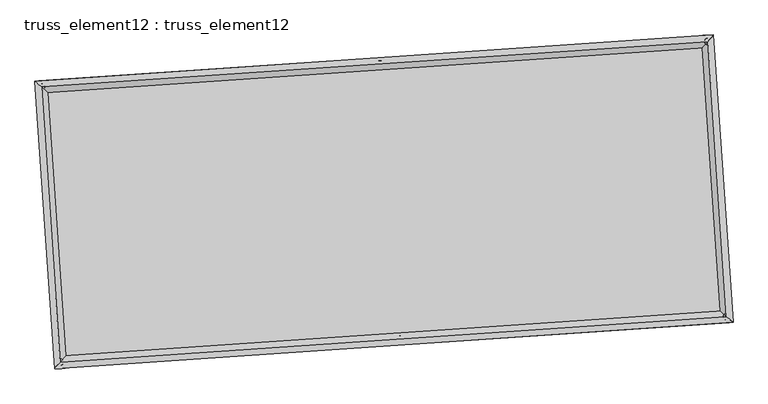
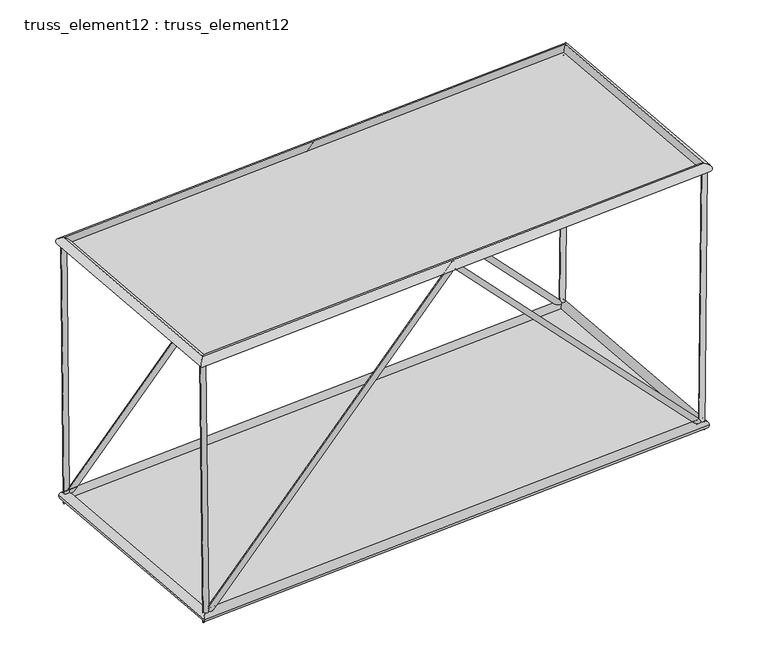
"""IFC4 building model written with IfcOpenShell, lengths in millimetres: plate geometry, truss_element12 : truss_element12."""

import ifcopenshell
import ifcopenshell.guid

model = None  # the IFC model being written
_history = None  # IfcOwnerHistory: only IFC2X3 demands one
_inside = {}  # id of a spatial element -> (the spatial element, [elements in it])
_under = {}  # id of a project, library or spatial element -> (it, [spatial elements below it])
_declared = {}  # id of a project -> (the project, [libraries it declares])
_typed = {}  # id of a type object -> (the type object, [elements of that type])
_made_of = {}  # id of a material, layer set ... -> (it, [elements and type objects made of it])


def new_model(schema):
    """Start an empty IFC model of exactly this schema.

    Asked for "IFC4X3", IfcOpenShell would pick the latest addendum, in which some entities
    have other attributes; the version numbers below select the first issue.
    IFC2X3 requires an IfcOwnerHistory on every rooted entity: one is made here for all.
    """
    global model, _history
    if schema == "IFC4X3":
        model = ifcopenshell.file(schema_version=(4, 3, 0, 0))
    else:
        model = ifcopenshell.file(schema=schema)
    _inside.clear()
    _under.clear()
    _declared.clear()
    _typed.clear()
    _made_of.clear()
    _history = None
    if model.schema == "IFC2X3":
        org = make("IfcOrganization", Name="unknown")
        user = make(
            "IfcPersonAndOrganization",
            ThePerson=make("IfcPerson", FamilyName="unknown"),
            TheOrganization=org,
        )
        app = make(
            "IfcApplication",
            ApplicationDeveloper=org,
            Version="unknown",
            ApplicationFullName="unknown",
            ApplicationIdentifier="unknown",
        )
        _history = make(
            "IfcOwnerHistory",
            OwningUser=user,
            OwningApplication=app,
            ChangeAction="ADDED",
            CreationDate=0,
        )
    return model


def make(cls, **values):
    """One entity of the class cls with the attributes given. An attribute that is None is left unset."""
    return model.create_entity(
        cls, **{name: value for name, value in values.items() if value is not None}
    )


def rooted(cls, **values):
    """An entity with a GlobalId (a new one), such as an element, a storey or a relation."""
    return make(cls, GlobalId=ifcopenshell.guid.new(), OwnerHistory=_history, **values)


def si_unit(unit_type, name, prefix=None):
    """IfcSIUnit, for example si_unit("LENGTHUNIT", "METRE", prefix="MILLI")."""
    return make("IfcSIUnit", UnitType=unit_type, Prefix=prefix, Name=name)


def assignment(units):
    """IfcUnitAssignment: the units of a project."""
    return None if units is None else make("IfcUnitAssignment", Units=units)


def point(xyz):
    """IfcCartesianPoint."""
    return None if xyz is None else make("IfcCartesianPoint", Coordinates=xyz)


def direction(xyz):
    """IfcDirection."""
    return None if xyz is None else make("IfcDirection", DirectionRatios=xyz)


def frame(location, z_axis=None, x_axis=None):
    """IfcAxis2Placement3D, a coordinate frame: its origin and axes. An axis left out is left unset."""
    return make(
        "IfcAxis2Placement3D",
        Location=point(location),
        Axis=direction(z_axis),
        RefDirection=direction(x_axis),
    )


def origin():
    """The frame at (0, 0, 0) with its axes left unset."""
    return frame((0.0, 0.0, 0.0))


def origin_with_axes():
    """The frame at (0, 0, 0) with the z axis (0, 0, 1) and the x axis (1, 0, 0) written out."""
    return frame((0.0, 0.0, 0.0), z_axis=(0.0, 0.0, 1.0), x_axis=(1.0, 0.0, 0.0))


def place(relative_to, where):
    """IfcLocalPlacement: puts the frame where relative to a parent placement (None: the world)."""
    return make(
        "IfcLocalPlacement", PlacementRelTo=relative_to, RelativePlacement=where
    )


def context(
    kind, dimensions, precision=None, world=None, true_north=None, identifier=None
):
    """IfcGeometricRepresentationContext, for example the 3D "Model" context."""
    return make(
        "IfcGeometricRepresentationContext",
        ContextIdentifier=identifier,
        ContextType=kind,
        CoordinateSpaceDimension=dimensions,
        Precision=precision,
        WorldCoordinateSystem=world,
        TrueNorth=true_north,
    )


def project(units=None, contexts=None):
    """IfcProject with its units and contexts."""
    return rooted(
        "IfcProject",
        Name="project",
        RepresentationContexts=contexts,
        UnitsInContext=assignment(units),
    )


def spatial(cls, under=None, at=None, **own):
    """A site, building, storey or space (cls), placed at a placement, below another one or the project."""
    s = rooted(cls, ObjectPlacement=at, **own)
    if under is not None:
        _under.setdefault(under.id(), (under, []))[1].append(s)
    return s


def polyline(points):
    """IfcPolyline through the points."""
    return make("IfcPolyline", Points=[point(p) for p in points])


def circle_curve(where, radius):
    """IfcCircle in the frame where."""
    return make("IfcCircle", Position=where, Radius=radius)


def ellipse_curve(where, semi_axis1, semi_axis2):
    """IfcEllipse in the frame where."""
    return make(
        "IfcEllipse", Position=where, SemiAxis1=semi_axis1, SemiAxis2=semi_axis2
    )


def outline(outer, holes=None, kind="AREA"):
    """IfcArbitraryClosedProfileDef: a profile drawn as a closed curve; with holes, ...WithVoids."""
    if holes is None:
        return make("IfcArbitraryClosedProfileDef", ProfileType=kind, OuterCurve=outer)
    return make(
        "IfcArbitraryProfileDefWithVoids",
        ProfileType=kind,
        OuterCurve=outer,
        InnerCurves=holes,
    )


def extrude(swept, where, along, depth):
    """IfcExtrudedAreaSolid: the profile swept, set in the frame where, extruded along a direction by depth."""
    return make(
        "IfcExtrudedAreaSolid",
        SweptArea=swept,
        Position=where,
        ExtrudedDirection=direction(along),
        Depth=depth,
    )


def shape(context_of_items, identifier, shape_type, items):
    """IfcShapeRepresentation: the items that make up one representation, for example the "Body"."""
    return make(
        "IfcShapeRepresentation",
        ContextOfItems=context_of_items,
        RepresentationIdentifier=identifier,
        RepresentationType=shape_type,
        Items=items,
    )


def source(mapping_origin, context_of_items, identifier, shape_type, items):
    """IfcRepresentationMap: a shape defined once, which mapped items show again and again."""
    return make(
        "IfcRepresentationMap",
        MappingOrigin=mapping_origin,
        MappedRepresentation=shape(context_of_items, identifier, shape_type, items),
    )


def transform(
    local_origin,
    x_axis=None,
    y_axis=None,
    z_axis=None,
    scale=None,
    scale2=None,
    scale3=None,
    uniform=True,
):
    """IfcCartesianTransformationOperator3D, or its non-uniform kind. x_axis, y_axis, z_axis: its Axis1, 2, 3."""
    if uniform:
        return make(
            "IfcCartesianTransformationOperator3D",
            Axis1=direction(x_axis),
            Axis2=direction(y_axis),
            LocalOrigin=point(local_origin),
            Scale=scale,
            Axis3=direction(z_axis),
        )
    return make(
        "IfcCartesianTransformationOperator3DnonUniform",
        Axis1=direction(x_axis),
        Axis2=direction(y_axis),
        LocalOrigin=point(local_origin),
        Scale=scale,
        Axis3=direction(z_axis),
        Scale2=scale2,
        Scale3=scale3,
    )


def mapped(mapping_source, mapping_target):
    """IfcMappedItem: shows the shape of a source again, moved by a transform."""
    return make(
        "IfcMappedItem", MappingSource=mapping_source, MappingTarget=mapping_target
    )


def made_of(thing, what):
    """Note that an element or type object is made of a material, layer set ...; save() writes the relation."""
    if what is not None:
        _made_of.setdefault(what.id(), (what, []))[1].append(thing)
    return thing


def element(
    cls,
    number,
    at=None,
    inside=None,
    cuts=None,
    type_object=None,
    material=None,
    context=None,
    identifier="Body",
    shape_type=None,
    held_by="IfcProductDefinitionShape",
    body=None,
    shapes=None,
    **own,
):
    """One element of the class cls, such as IfcWall. Its Tag is "e" and its number.

    at: its placement. inside: the storey or other place that contains it. cuts: it is an
    opening in that element (IfcRelVoidsElement). A single representation is given by context,
    identifier, shape_type and body (its items); several are given by shapes. held_by: the class
    of the entity that holds the representations. save() writes the other relations.
    """
    e = rooted(cls, Tag="e%d" % number, ObjectPlacement=at, **own)
    if body is not None:
        shapes = [shape(context, identifier, shape_type, body)]
    if shapes is not None:
        e.Representation = make(held_by, Representations=shapes)
    if inside is not None:
        _inside.setdefault(inside.id(), (inside, []))[1].append(e)
    if cuts is not None:
        rooted(
            "IfcRelVoidsElement", RelatingBuildingElement=cuts, RelatedOpeningElement=e
        )
    if type_object is not None:
        _typed.setdefault(type_object.id(), (type_object, []))[1].append(e)
    return made_of(e, material)


def aggregate(whole, parts):
    """IfcRelAggregates: a whole, such as a stair, and the parts it consists of."""
    return rooted("IfcRelAggregates", RelatingObject=whole, RelatedObjects=parts)


def save(model, path):
    """Write the relations noted so far, then the file.

    IfcRelAggregates (storeys below a building ...), IfcRelContainedInSpatialStructure (elements
    in a storey), IfcRelDefinesByType, IfcRelAssociatesMaterial and IfcRelDeclares: one each for
    every whole, place, type object, material and project.
    """
    for whole, parts in _under.values():
        aggregate(whole, parts)
    for where, things in _inside.values():
        rooted(
            "IfcRelContainedInSpatialStructure",
            RelatedElements=things,
            RelatingStructure=where,
        )
    for kind, things in _typed.values():
        rooted("IfcRelDefinesByType", RelatedObjects=things, RelatingType=kind)
    for what, things in _made_of.values():
        rooted("IfcRelAssociatesMaterial", RelatedObjects=things, RelatingMaterial=what)
    for by, libraries in _declared.values():
        rooted("IfcRelDeclares", RelatingContext=by, RelatedDefinitions=libraries)
    model.write(path)


def plane_surface(at):
    """IfcPlane: the flat surface through the origin of the frame at, square to its z axis."""
    return make("IfcPlane", Position=at)


def cylinder_surface(at, radius):
    """IfcCylindricalSurface: all points at the distance radius from the z axis of the frame at."""
    return make("IfcCylindricalSurface", Position=at, Radius=radius)


def advanced_brep(points, edges, surfaces, faces):
    """IfcAdvancedBrep: a solid bounded by faces that lie on surfaces and meet in shared edges.

    An edge is (start, end): straight between two places in points (the first is 0);
    or (start, end, curve); or (start, end, curve, False) where it runs against its curve.
    A face is (place in surfaces, loops), or (place, loops, False) where it looks against
    its surface's normal. A loop lists edges by number (the first is 1), with a minus sign
    where the edge is run from its end to its start. The first loop is the outer one.
    """
    corners = [point(p) for p in points]
    vertices = [make("IfcVertexPoint", VertexGeometry=c) for c in corners]
    made = []
    for start, end, *more in edges:
        made.append(
            make(
                "IfcEdgeCurve",
                EdgeStart=vertices[start],
                EdgeEnd=vertices[end],
                EdgeGeometry=more[0] if more else make("IfcPolyline", Points=[corners[start], corners[end]]),
                SameSense=more[1] if len(more) > 1 else True,
            )
        )
    hull = []
    for where, loops, *sense in faces:
        bounds = []
        for j, loop in enumerate(loops):
            ring = [make("IfcOrientedEdge", EdgeElement=made[abs(k) - 1], Orientation=k > 0) for k in loop]
            bounds.append(
                make(
                    "IfcFaceOuterBound" if j == 0 else "IfcFaceBound",
                    Bound=make("IfcEdgeLoop", EdgeList=ring),
                    Orientation=True,
                )
            )
        hull.append(make("IfcAdvancedFace", Bounds=bounds, FaceSurface=surfaces[where], SameSense=sense[0] if sense else True))
    return make("IfcAdvancedBrep", Outer=make("IfcClosedShell", CfsFaces=hull))


def truss_element12_truss_element12_25fafcbe(model_context):
    return source(origin(), model_context, "Body", "SolidModel", [
        advanced_brep(
        [(-3717.9336518, 2272.6106472, 5000.2478695), (-3817.0314009, 2259.2497843, 4999.187935), (-3666.2408019, 2276.1353862, 122.8345798), (-3762.7460809, 2262.9512939, -122.8345798), (1064.197845, 2598.6860154, 5071.8345971), (1064.6389029, 2592.1123254, 4927.5910047), (5793.7028088, 2921.1729804, 122.8278987), (5891.0581682, 2921.2075081, -122.8278987), (5846.3222996, 2924.7609034, 5000.2471651), (5946.316249, 2924.9753466, 4999.1682339)],
        [
            (0, 1, circle_curve(frame((-3767.4825264, 2265.9302158, 4999.7179023), z_axis=(-0.01059781698674716, -0.0007226248542523914, 0.9999435804526352), x_axis=(-0.13360875038090175, 0.9910339106331651, -0.0006998548346273042)), 50.0)),
            (1, 0, circle_curve(frame((-3767.4825264, 2265.9302158, 4999.7179023), z_axis=(-0.01059781698674716, -0.0007226248542523914, 0.9999435804526352), x_axis=(-0.13360875038090175, 0.9910339106331651, -0.0006998548346273042)), 50.0)),
            (0, 2),
            (2, 3, ellipse_curve(frame((-3714.4934414, 2269.54334, 0.0), z_axis=(-0.9277371610449594, -0.06325887035254743, 0.36783430418866414), x_axis=(0.36698217779578546, 0.025023119674036753, 0.9298913509986214)), 132.383262, 50.0)),
            (3, 1),
            (3, 2, ellipse_curve(frame((-3714.4934414, 2269.54334, 0.0), z_axis=(-0.9277371610449594, -0.06325887035254743, 0.36783430418866414), x_axis=(0.36698217779578546, 0.025023119674036753, 0.9298913509986214)), 132.383262, 50.0)),
            (2, 4),
            (4, 5, ellipse_curve(frame((1064.418374, 2595.3991704, 4999.7128009), z_axis=(-0.9976833948456157, -0.0680282381448872, 4.9641008010384885e-05), x_axis=(-4.952600945652472e-05, -3.3769903190067476e-06, -0.9999999987678853)), 72.2788404, 50.0)),
            (5, 3),
            (5, 4, ellipse_curve(frame((1064.418374, 2595.3991704, 4999.7128009), z_axis=(-0.9976833948456157, -0.0680282381448872, 4.9641008010384885e-05), x_axis=(-4.952600945652472e-05, -3.3769903190067476e-06, -0.9999999987678853)), 72.2788404, 50.0)),
            (4, 6),
            (6, 7, ellipse_curve(frame((5842.3804885, 2921.1902443, 0.0), z_axis=(-0.9277903039426281, -0.06326249396472418, -0.36769961757854613), x_axis=(-0.3668478032011972, -0.025013957181237265, 0.9299446172931972)), 132.3684791, 50.0)),
            (7, 5),
            (7, 6, ellipse_curve(frame((5842.3804885, 2921.1902443, 0.0), z_axis=(-0.9277903039426281, -0.06326249396472418, -0.36769961757854613), x_axis=(-0.3668478032011972, -0.025013957181237265, 0.9299446172931972)), 132.3684791, 50.0)),
            (8, 9, circle_curve(frame((5896.3192743, 2924.868125, 4999.7076995), z_axis=(0.010787757166797024, 0.0007355761530998497, 0.9999415399027252), x_axis=(-0.0021522428826436795, 0.9999974301665041, -0.0007123980360681724)), 50.0)),
            (9, 8, circle_curve(frame((5896.3192743, 2924.868125, 4999.7076995), z_axis=(0.010787757166797024, 0.0007355761530998497, 0.9999415399027252), x_axis=(-0.0021522428826436795, 0.9999974301665041, -0.0007123980360681724)), 50.0)),
            (6, 8),
            (9, 7),
        ],
        [
            plane_surface(frame((-3767.4825264, 2315.9302027, 4999.7540355), z_axis=(-0.010597816986746694, -0.0007226248542495527, 0.9999435804526353), x_axis=(0.9999438415606726, -7.658676055122278e-06, 0.010597814219416088))),
            cylinder_surface(frame((-3767.4825264, 2265.9302158, 4999.7179023), z_axis=(-0.01059781698674716, -0.0007226248542523914, 0.9999435804526352), x_axis=(-0.13360875038090175, 0.9910339106331651, -0.0006998548346273042)), 50.0),
            cylinder_surface(frame((-3714.4934414, 2269.54334, 0.0), z_axis=(-0.6901986031859024, -0.04706201906073101, -0.7220879825354779), x_axis=(-0.020416121080295117, 0.9987520857397071, -0.045579087645757826)), 50.0),
            cylinder_surface(frame((1064.418374, 2595.3991704, 4999.7128009), z_axis=(-0.690127075511872, -0.04705714186054079, 0.7221566623976738), x_axis=(-0.11534925252048381, 0.9922789563814176, -0.04557436412689142)), 50.0),
            plane_surface(frame((5896.3192743, 2874.8681385, 4999.7444805), z_axis=(0.010787757166796641, 0.0007355761530995457, 0.9999415399027253), x_axis=(0.9999418104546436, -7.935678690174086e-06, -0.010787754247978398))),
            cylinder_surface(frame((5842.3804885, 2921.1902443, 0.0), z_axis=(-0.010787757166797024, -0.0007355761530998497, -0.9999415399027252), x_axis=(-0.0021522428826436795, 0.9999974301665041, -0.0007123980360681724)), 50.0),
        ],
        [
            (0, [[1, 2]]),
            (1, [[-1, 3, 4, 5]]),
            (1, [[-2, -5, 6, -3]]),
            (2, [[-4, 7, 8, 9]]),
            (2, [[-6, -9, 10, -7]]),
            (3, [[-8, 11, 12, 13]]),
            (3, [[-10, -13, 14, -11]]),
            (4, [[15, 16]]),
            (5, [[-12, 17, -16, 18]]),
            (5, [[-14, -18, -15, -17]]),
        ],
    ),
        advanced_brep(
        [(-3445.8206989, -1718.1229371, 5000.2478695), (-3544.918448, -1731.4838, 4999.187935), (-3394.127849, -1714.5981981, 122.8345798), (-3490.633128, -1727.7822904, -122.8345798), (1336.310798, -1392.0475689, 5071.8345971), (1336.7518559, -1398.6212589, 4927.5910047), (6065.8157618, -1069.5606039, 122.8278987), (6163.1711211, -1069.5260762, -122.8278987), (6118.4352525, -1065.9726809, 5000.2471651), (6218.429202, -1065.7582377, 4999.1682339)],
        [
            (0, 1, circle_curve(frame((-3495.3695734, -1724.8033685, 4999.7179023), z_axis=(-0.01059781698674734, -0.0007226248542523697, 0.9999435804526352), x_axis=(-0.13360875038090145, 0.9910339106331651, -0.000699854834627346)), 50.0)),
            (1, 0, circle_curve(frame((-3495.3695734, -1724.8033685, 4999.7179023), z_axis=(-0.01059781698674734, -0.0007226248542523697, 0.9999435804526352), x_axis=(-0.13360875038090145, 0.9910339106331651, -0.000699854834627346)), 50.0)),
            (0, 2),
            (2, 3, ellipse_curve(frame((-3442.3804885, -1721.1902443, 0.0), z_axis=(-0.9277371610449594, -0.06325887035254724, 0.3678343041886641), x_axis=(0.3669821777957854, 0.02502311967403671, 0.9298913509986214)), 132.383262, 50.0)),
            (3, 1),
            (3, 2, ellipse_curve(frame((-3442.3804885, -1721.1902443, 0.0), z_axis=(-0.9277371610449594, -0.06325887035254724, 0.3678343041886641), x_axis=(0.3669821777957854, 0.02502311967403671, 0.9298913509986214)), 132.383262, 50.0)),
            (2, 4),
            (4, 5, ellipse_curve(frame((1336.5313269, -1395.3344139, 4999.7128009), z_axis=(-0.9976833948456157, -0.06802823814488712, 4.964100801046513e-05), x_axis=(-4.952600945652472e-05, -3.3769903189394843e-06, -0.9999999987678853)), 72.2788404, 50.0)),
            (5, 3),
            (5, 4, ellipse_curve(frame((1336.5313269, -1395.3344139, 4999.7128009), z_axis=(-0.9976833948456157, -0.06802823814488712, 4.964100801046513e-05), x_axis=(-4.952600945652472e-05, -3.3769903189394843e-06, -0.9999999987678853)), 72.2788404, 50.0)),
            (4, 6),
            (6, 7, ellipse_curve(frame((6114.4934414, -1069.54334, 0.0), z_axis=(-0.9277903039426281, -0.06326249396472412, -0.3676996175785463), x_axis=(-0.36684780320119736, -0.025013957181237296, 0.9299446172931972)), 132.3684791, 50.0)),
            (7, 5),
            (7, 6, ellipse_curve(frame((6114.4934414, -1069.54334, 0.0), z_axis=(-0.9277903039426281, -0.06326249396472412, -0.3676996175785463), x_axis=(-0.36684780320119736, -0.025013957181237296, 0.9299446172931972)), 132.3684791, 50.0)),
            (8, 9, circle_curve(frame((6168.4322273, -1065.8654593, 4999.7076995), z_axis=(0.010787757166797012, 0.00073557615309981, 0.9999415399027253), x_axis=(-0.0021522428826438933, 0.9999974301665041, -0.0007123980360681303)), 50.0)),
            (9, 8, circle_curve(frame((6168.4322273, -1065.8654593, 4999.7076995), z_axis=(0.010787757166797012, 0.00073557615309981, 0.9999415399027253), x_axis=(-0.0021522428826438933, 0.9999974301665041, -0.0007123980360681303)), 50.0)),
            (6, 8),
            (9, 7),
        ],
        [
            plane_surface(frame((-3495.3695734, -1674.8033816, 4999.7540355), z_axis=(-0.010597816986746694, -0.0007226248542495488, 0.9999435804526353), x_axis=(0.9999438415606726, -7.658676055122278e-06, 0.010597814219416088))),
            cylinder_surface(frame((-3495.3695734, -1724.8033685, 4999.7179023), z_axis=(-0.01059781698674734, -0.0007226248542523697, 0.9999435804526352), x_axis=(-0.13360875038090145, 0.9910339106331651, -0.000699854834627346)), 50.0),
            cylinder_surface(frame((-3442.3804885, -1721.1902443, 0.0), z_axis=(-0.6901986031859025, -0.0470620190607309, -0.7220879825354778), x_axis=(-0.0204161210802951, 0.9987520857397071, -0.0455790876457577)), 50.0),
            cylinder_surface(frame((1336.5313269, -1395.3344139, 4999.7128009), z_axis=(-0.6901270755118721, -0.047057141860540795, 0.722156662397674), x_axis=(-0.11534925252048368, 0.9922789563814176, -0.0455743641268913)), 50.0),
            plane_surface(frame((6168.4322273, -1115.8654458, 4999.7444805), z_axis=(0.010787757166796641, 0.0007355761530995437, 0.9999415399027253), x_axis=(0.9999418104546436, -7.935678691062265e-06, -0.010787754247978398))),
            cylinder_surface(frame((6114.4934414, -1069.54334, 0.0), z_axis=(-0.010787757166797012, -0.00073557615309981, -0.9999415399027253), x_axis=(-0.0021522428826438933, 0.9999974301665041, -0.0007123980360681303)), 50.0),
        ],
        [
            (0, [[1, 2]]),
            (1, [[-1, 3, 4, 5]]),
            (1, [[-2, -5, 6, -3]]),
            (2, [[-4, 7, 8, 9]]),
            (2, [[-6, -9, 10, -7]]),
            (3, [[-8, 11, 12, 13]]),
            (3, [[-10, -13, 14, -11]]),
            (4, [[15, 16]]),
            (5, [[-12, 17, -16, 18]]),
            (5, [[-14, -18, -15, -17]]),
        ],
    ),
        advanced_brep(
        [(-3495.372256, -1724.8063417, 4909.7179023), (-3495.3668909, -1724.8003953, 5089.7179022), (-3767.479465, 2265.9276342, 5089.7179022), (-3767.4855877, 2265.9327973, 4909.7179023), (5896.3167809, 2924.8651647, 5089.7076995), (5896.3217678, 2924.8710853, 4909.7076996), (6168.4293551, -1065.8628648, 5089.7076995), (6168.4350994, -1065.8680537, 4909.7076996)],
        [
            (0, 1, ellipse_curve(frame((-3495.3695734, -1724.8033685, 4999.7179023), z_axis=(-0.7535719234050675, 0.6573654662781063, 7.448125025781954e-07), x_axis=(-0.6573654662776883, -0.7535719234054323, 7.448125025782821e-07)), 127.2792206, 90.0)),
            (1, 2),
            (2, 3, ellipse_curve(frame((-3767.4825264, 2265.9302158, 4999.7179023), z_axis=(-0.6573654662776883, -0.7535719234054322, 7.448125025783611e-07), x_axis=(0.7535719234050674, -0.6573654662781064, -7.44812502578274e-07)), 127.2792206, 90.0)),
            (3, 0),
            (1, 0, ellipse_curve(frame((-3495.3695734, -1724.8033685, 4999.7179023), z_axis=(-0.7535719234050675, 0.6573654662781063, 7.448125025781954e-07), x_axis=(-0.6573654662776883, -0.7535719234054323, 7.448125025782821e-07)), 127.2792206, 90.0)),
            (3, 2, ellipse_curve(frame((-3767.4825264, 2265.9302158, 4999.7179023), z_axis=(-0.6573654662776883, -0.7535719234054322, 7.448125025783611e-07), x_axis=(0.7535719234050674, -0.6573654662781064, -7.44812502578274e-07)), 127.2792206, 90.0)),
            (2, 4),
            (4, 5, ellipse_curve(frame((5896.3192743, 2924.868125, 4999.7076995), z_axis=(-0.7535719234050677, 0.6573654662781063, 7.448125025783542e-07), x_axis=(-0.6573654662776882, -0.7535719234054323, 7.448125025782813e-07)), 127.2792206, 90.0)),
            (5, 3),
            (5, 4, ellipse_curve(frame((5896.3192743, 2924.868125, 4999.7076995), z_axis=(-0.7535719234050677, 0.6573654662781063, 7.448125025783542e-07), x_axis=(-0.6573654662776882, -0.7535719234054323, 7.448125025782813e-07)), 127.2792206, 90.0)),
            (4, 6),
            (6, 7, ellipse_curve(frame((6168.4322273, -1065.8654593, 4999.7076995), z_axis=(0.6573654662776882, 0.7535719234054323, -7.448125025782022e-07), x_axis=(-0.7535719234050676, 0.6573654662781062, 7.448125025782751e-07)), 127.2792206, 90.0)),
            (7, 5),
            (7, 6, ellipse_curve(frame((6168.4322273, -1065.8654593, 4999.7076995), z_axis=(0.6573654662776882, 0.7535719234054323, -7.448125025782022e-07), x_axis=(-0.7535719234050676, 0.6573654662781062, 7.448125025782751e-07)), 127.2792206, 90.0)),
            (6, 1),
            (0, 7),
        ],
        [
            cylinder_surface(frame((-3495.3695734, -1724.8033685, 4999.7179023), z_axis=(0.06802823822870346, -0.9976833960748764, 0.0), x_axis=(-0.9976833955645505, -0.06802823819390627, 3.1984710746243846e-05)), 90.0),
            cylinder_surface(frame((-3767.4825264, 2265.9302158, 4999.7179023), z_axis=(-0.9976833960743232, -0.06802823822866429, 1.053323942571303e-06), x_axis=(-0.0680282381636537, 0.9976833955998259, 3.093138680417647e-05)), 90.0),
            cylinder_surface(frame((5896.3192743, 2924.868125, 4999.7076995), z_axis=(-0.06802823822870388, 0.9976833960748765, 0.0), x_axis=(0.9976833956295612, 0.06802823819833952, 2.9878062862109108e-05)), 90.0),
            cylinder_surface(frame((6168.4322273, -1065.8654593, 4999.7076995), z_axis=(0.9976833960743232, 0.06802823822866422, -1.0533239425711911e-06), x_axis=(0.06802823822866422, -0.9976833955953931, 3.093138680417647e-05)), 90.0),
        ],
        [
            (0, [[1, 2, 3, 4]]),
            (0, [[5, -4, 6, -2]]),
            (1, [[-3, 7, 8, 9]]),
            (1, [[-6, -9, 10, -7]]),
            (2, [[-8, 11, 12, 13]]),
            (2, [[-10, -13, 14, -11]]),
            (3, [[-12, 15, -1, 16]]),
            (3, [[-14, -16, -5, -15]]),
        ],
    ),
        advanced_brep(
        [(-3358.7115243, -1625.2761972, 0.0), (-3526.0494527, -1817.1042913, 0.0), (-3810.4074885, 2353.2123043, 0.0), (-3618.5793943, 2185.8743758, 0.0), (5926.0494527, 3017.1042913, 0.0), (5758.7115243, 2825.2761972, 0.0), (6210.4074885, -1153.2123043, 0.0), (6018.5793943, -985.8743758, 0.0)],
        [
            (0, 1, ellipse_curve(frame((-3442.3804885, -1721.1902443, 0.0), z_axis=(-0.7535719234054613, 0.6573654662780769, 0.0), x_axis=(-0.6573654662780767, -0.7535719234054614, 0.0)), 127.2792206, 90.0)),
            (1, 2),
            (2, 3, ellipse_curve(frame((-3714.4934414, 2269.54334, 0.0), z_axis=(-0.6573654662780768, -0.7535719234054614, 0.0), x_axis=(0.7535719234054613, -0.6573654662780768, 0.0)), 127.2792206, 90.0)),
            (3, 0),
            (1, 0, ellipse_curve(frame((-3442.3804885, -1721.1902443, 0.0), z_axis=(-0.7535719234054613, 0.6573654662780769, 0.0), x_axis=(-0.6573654662780767, -0.7535719234054614, 0.0)), 127.2792206, 90.0)),
            (3, 2, ellipse_curve(frame((-3714.4934414, 2269.54334, 0.0), z_axis=(-0.6573654662780768, -0.7535719234054614, 0.0), x_axis=(0.7535719234054613, -0.6573654662780768, 0.0)), 127.2792206, 90.0)),
            (2, 4),
            (4, 5, ellipse_curve(frame((5842.3804885, 2921.1902443, 0.0), z_axis=(-0.7535719234054613, 0.6573654662780768, 0.0), x_axis=(-0.657365466278077, -0.7535719234054612, 0.0)), 127.2792206, 90.0)),
            (5, 3),
            (5, 4, ellipse_curve(frame((5842.3804885, 2921.1902443, 0.0), z_axis=(-0.7535719234054613, 0.6573654662780768, 0.0), x_axis=(-0.657365466278077, -0.7535719234054612, 0.0)), 127.2792206, 90.0)),
            (4, 6),
            (6, 7, ellipse_curve(frame((6114.4934414, -1069.54334, 0.0), z_axis=(0.657365466278077, 0.7535719234054614, 0.0), x_axis=(-0.7535719234054615, 0.6573654662780768, 0.0)), 127.2792206, 90.0)),
            (7, 5),
            (7, 6, ellipse_curve(frame((6114.4934414, -1069.54334, 0.0), z_axis=(0.657365466278077, 0.7535719234054614, 0.0), x_axis=(-0.7535719234054615, 0.6573654662780768, 0.0)), 127.2792206, 90.0)),
            (6, 1),
            (0, 7),
        ],
        [
            cylinder_surface(frame((-3442.3804885, -1721.1902443, 0.0), z_axis=(0.06802823822870728, -0.9976833960748762, 0.0), x_axis=(-0.9976833960748762, -0.06802823822870728, 0.0)), 90.0),
            cylinder_surface(frame((-3714.4934414, 2269.54334, 0.0), z_axis=(-0.9976833960748763, -0.06802823822870568, 0.0), x_axis=(-0.06802823822870568, 0.9976833960748763, 0.0)), 90.0),
            cylinder_surface(frame((5842.3804885, 2921.1902443, 0.0), z_axis=(-0.0680282382287072, 0.9976833960748762, 0.0), x_axis=(0.9976833960748762, 0.0680282382287072, 0.0)), 90.0),
            cylinder_surface(frame((6114.4934414, -1069.54334, 0.0), z_axis=(0.9976833960748763, 0.0680282382287056, 0.0), x_axis=(0.0680282382287056, -0.9976833960748763, 0.0)), 90.0),
        ],
        [
            (0, [[1, 2, 3, 4]]),
            (0, [[5, -4, 6, -2]]),
            (1, [[-3, 7, 8, 9]]),
            (1, [[-6, -9, 10, -7]]),
            (2, [[-8, 11, 12, 13]]),
            (2, [[-10, -13, 14, -11]]),
            (3, [[-12, 15, -1, 16]]),
            (3, [[-14, -16, -5, -15]]),
        ],
    ),
        extrude(outline(polyline([(-3442.3804885, -1721.1902443), (-3714.4934414, 2269.54334), (5842.3804885, 2921.1902443), (6114.4934414, -1069.54334), (-3442.3804885, -1721.1902443)])), origin_with_axes(), (0.0, 0.0, 1.0), 20.0),
        extrude(outline(polyline([(-1999.9999999, 4843.1204923), (2000.0000001, 4843.1204924), (2000.0, -4843.1204922), (-2000.0, -4843.1204923), (-1999.9999999, 4843.1204923)])), frame((1200.4748505, 600.0323782, 4999.7128009), z_axis=(1.0508838081914596e-06, 7.165577209723778e-08, 0.9999999999994453), x_axis=(-0.06802823822870709, 0.9976833960748762, 0.0)), (0.0, 0.0, 1.0), 20.0),
    ])


if __name__ == "__main__":
    model = new_model("IFC4")
    model_context = context("Model", 3, world=origin())
    ifc_project = project(units=[si_unit("LENGTHUNIT", "METRE", prefix="MILLI")], contexts=[model_context])
    site = spatial("IfcSite", under=ifc_project)
    building = spatial("IfcBuilding", under=site)
    placement = place(None, origin())
    truss_element12_truss_element12_shape = truss_element12_truss_element12_25fafcbe(model_context)
    element("IfcPlate", 1, ObjectType="truss_element12 : truss_element12", at=placement, inside=building, context=model_context, shape_type="MappedRepresentation", body=[
        mapped(truss_element12_truss_element12_shape, transform((0.0, 0.0, 0.0), x_axis=(1.0, 0.0, 0.0), y_axis=(0.0, 1.0, 0.0), z_axis=(0.0, 0.0, 1.0))),
    ])
    save(model, "model.ifc")

# Revit data of these elements
# Type "truss_element12 : truss_element12"
#   steellbar1 = 90 mm
#   steelbar2 = 50 mm
#   offset1 = 5000 mm
#   M = Default Roof
# Element 1 (IfcPlate, "truss_element12 : truss_element12")
#   Materials on its faces: "Default Roof"
# Materials
#   "Default Roof": class "Miscellaneous", colour RGB 0 127 0, transparency 0, Comments = "Rendering appearance not upgraded Rendering appearance not upgraded ", Cost = 0
